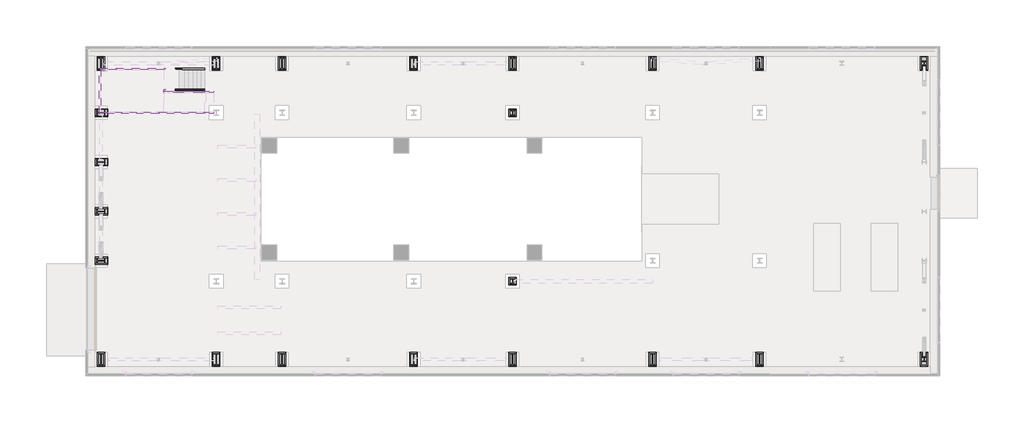
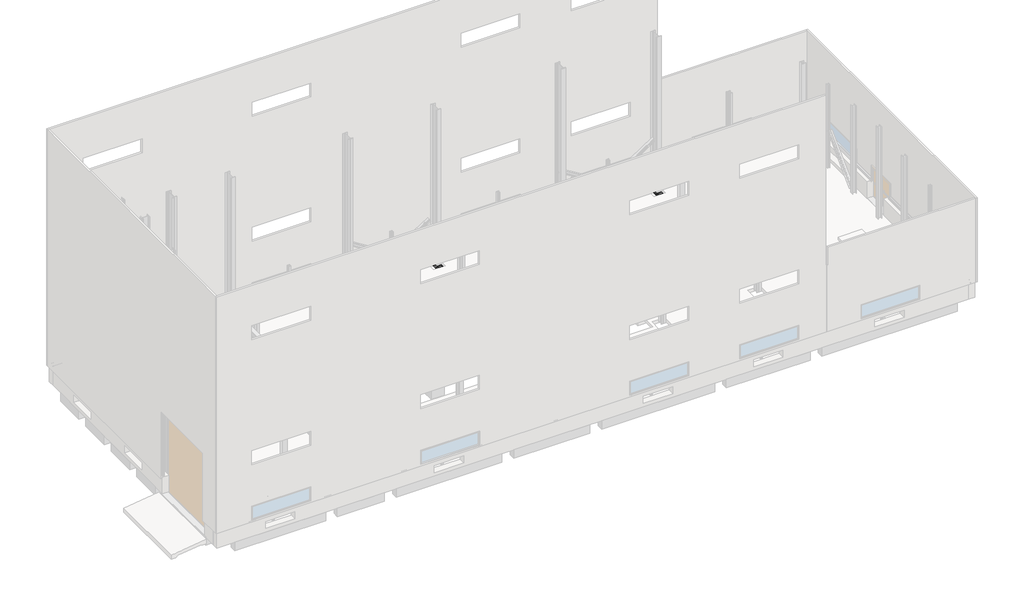
# One storey, part 4 of 4: 23 proxies, 10 members.
"""IFC4 building model written with IfcOpenShell, lengths in millimetres."""

import ifcopenshell
import ifcopenshell.guid

model = None  # the IFC model being written
_history = None  # IfcOwnerHistory: only IFC2X3 demands one
_inside = {}  # id of a spatial element -> (the spatial element, [elements in it])
_under = {}  # id of a project, library or spatial element -> (it, [spatial elements below it])
_declared = {}  # id of a project -> (the project, [libraries it declares])
_typed = {}  # id of a type object -> (the type object, [elements of that type])
_made_of = {}  # id of a material, layer set ... -> (it, [elements and type objects made of it])


def new_model(schema):
    """Start an empty IFC model of exactly this schema.

    Asked for "IFC4X3", IfcOpenShell would pick the latest addendum, in which some entities
    have other attributes; the version numbers below select the first issue.
    IFC2X3 requires an IfcOwnerHistory on every rooted entity: one is made here for all.
    """
    global model, _history
    if schema == "IFC4X3":
        model = ifcopenshell.file(schema_version=(4, 3, 0, 0))
    else:
        model = ifcopenshell.file(schema=schema)
    _inside.clear()
    _under.clear()
    _declared.clear()
    _typed.clear()
    _made_of.clear()
    _history = None
    if model.schema == "IFC2X3":
        org = make("IfcOrganization", Name="unknown")
        user = make(
            "IfcPersonAndOrganization",
            ThePerson=make("IfcPerson", FamilyName="unknown"),
            TheOrganization=org,
        )
        app = make(
            "IfcApplication",
            ApplicationDeveloper=org,
            Version="unknown",
            ApplicationFullName="unknown",
            ApplicationIdentifier="unknown",
        )
        _history = make(
            "IfcOwnerHistory",
            OwningUser=user,
            OwningApplication=app,
            ChangeAction="ADDED",
            CreationDate=0,
        )
    return model


def make(cls, **values):
    """One entity of the class cls with the attributes given. An attribute that is None is left unset."""
    return model.create_entity(
        cls, **{name: value for name, value in values.items() if value is not None}
    )


def rooted(cls, **values):
    """An entity with a GlobalId (a new one), such as an element, a storey or a relation."""
    return make(cls, GlobalId=ifcopenshell.guid.new(), OwnerHistory=_history, **values)


def si_unit(unit_type, name, prefix=None):
    """IfcSIUnit, for example si_unit("LENGTHUNIT", "METRE", prefix="MILLI")."""
    return make("IfcSIUnit", UnitType=unit_type, Prefix=prefix, Name=name)


def assignment(units):
    """IfcUnitAssignment: the units of a project."""
    return None if units is None else make("IfcUnitAssignment", Units=units)


def point(xyz):
    """IfcCartesianPoint."""
    return None if xyz is None else make("IfcCartesianPoint", Coordinates=xyz)


def direction(xyz):
    """IfcDirection."""
    return None if xyz is None else make("IfcDirection", DirectionRatios=xyz)


def frame(location, z_axis=None, x_axis=None):
    """IfcAxis2Placement3D, a coordinate frame: its origin and axes. An axis left out is left unset."""
    return make(
        "IfcAxis2Placement3D",
        Location=point(location),
        Axis=direction(z_axis),
        RefDirection=direction(x_axis),
    )


def frame_2d(location, x_axis=None):
    """IfcAxis2Placement2D, a coordinate frame in the plane: its origin and x axis."""
    return make(
        "IfcAxis2Placement2D", Location=point(location), RefDirection=direction(x_axis)
    )


def origin():
    """The frame at (0, 0, 0) with its axes left unset."""
    return frame((0.0, 0.0, 0.0))


def place(relative_to, where):
    """IfcLocalPlacement: puts the frame where relative to a parent placement (None: the world)."""
    return make(
        "IfcLocalPlacement", PlacementRelTo=relative_to, RelativePlacement=where
    )


def context(
    kind, dimensions, precision=None, world=None, true_north=None, identifier=None
):
    """IfcGeometricRepresentationContext, for example the 3D "Model" context."""
    return make(
        "IfcGeometricRepresentationContext",
        ContextIdentifier=identifier,
        ContextType=kind,
        CoordinateSpaceDimension=dimensions,
        Precision=precision,
        WorldCoordinateSystem=world,
        TrueNorth=true_north,
    )


def project(units=None, contexts=None):
    """IfcProject with its units and contexts."""
    return rooted(
        "IfcProject",
        Name="project",
        RepresentationContexts=contexts,
        UnitsInContext=assignment(units),
    )


def spatial(cls, under=None, at=None, **own):
    """A site, building, storey or space (cls), placed at a placement, below another one or the project."""
    s = rooted(cls, ObjectPlacement=at, **own)
    if under is not None:
        _under.setdefault(under.id(), (under, []))[1].append(s)
    return s


def polyline(points):
    """IfcPolyline through the points."""
    return make("IfcPolyline", Points=[point(p) for p in points])


def circle_curve(where, radius):
    """IfcCircle in the frame where."""
    return make("IfcCircle", Position=where, Radius=radius)


def ellipse_curve(where, semi_axis1, semi_axis2):
    """IfcEllipse in the frame where."""
    return make(
        "IfcEllipse", Position=where, SemiAxis1=semi_axis1, SemiAxis2=semi_axis2
    )


def trimmed(basis, trim1, trim2, sense, master):
    """IfcTrimmedCurve: the piece of a basis curve between two trims."""
    return make(
        "IfcTrimmedCurve",
        BasisCurve=basis,
        Trim1=trim1,
        Trim2=trim2,
        SenseAgreement=sense,
        MasterRepresentation=master,
    )


def segment(curve, same_sense, transition):
    """IfcCompositeCurveSegment."""
    return make(
        "IfcCompositeCurveSegment",
        Transition=transition,
        SameSense=same_sense,
        ParentCurve=curve,
    )


def composite_curve(segments, self_intersect=None):
    """IfcCompositeCurve: segments joined end to end."""
    return make("IfcCompositeCurve", Segments=segments, SelfIntersect=self_intersect)


def outline(outer, holes=None, kind="AREA"):
    """IfcArbitraryClosedProfileDef: a profile drawn as a closed curve; with holes, ...WithVoids."""
    if holes is None:
        return make("IfcArbitraryClosedProfileDef", ProfileType=kind, OuterCurve=outer)
    return make(
        "IfcArbitraryProfileDefWithVoids",
        ProfileType=kind,
        OuterCurve=outer,
        InnerCurves=holes,
    )


def extrude(swept, where, along, depth):
    """IfcExtrudedAreaSolid: the profile swept, set in the frame where, extruded along a direction by depth."""
    return make(
        "IfcExtrudedAreaSolid",
        SweptArea=swept,
        Position=where,
        ExtrudedDirection=direction(along),
        Depth=depth,
    )


def faces_of(points, faces, orient=None, outer=None):
    """IfcFace entities. A face is a list of loops; a loop is a list of indices into points, from 0.

    orient and outer hold one flag for each loop. By default every Orientation is true, the
    first loop of a face is its IfcFaceOuterBound and the others are IfcFaceBound.
    """
    made = []
    for i, loops in enumerate(faces):
        bounds = []
        for j, loop in enumerate(loops):
            is_outer = j == 0 if outer is None else outer[i][j]
            bounds.append(
                make(
                    "IfcFaceOuterBound" if is_outer else "IfcFaceBound",
                    Bound=make("IfcPolyLoop", Polygon=[points[k] for k in loop]),
                    Orientation=True if orient is None else orient[i][j],
                )
            )
        made.append(make("IfcFace", Bounds=bounds))
    return made


def faceted_brep(points, faces, orient=None, outer=None, voids=None):
    """IfcFacetedBrep: a solid bounded by flat faces; with voids (closed shells), ...WithVoids."""
    shared = [point(p) for p in points]
    hull = make("IfcClosedShell", CfsFaces=faces_of(shared, faces, orient, outer))
    if voids is None:
        return make("IfcFacetedBrep", Outer=hull)
    return make(
        "IfcFacetedBrepWithVoids",
        Outer=hull,
        Voids=[
            make(cls, CfsFaces=faces_of(shared, fs, o, b)) for cls, fs, o, b in voids
        ],
    )


def shape(context_of_items, identifier, shape_type, items):
    """IfcShapeRepresentation: the items that make up one representation, for example the "Body"."""
    return make(
        "IfcShapeRepresentation",
        ContextOfItems=context_of_items,
        RepresentationIdentifier=identifier,
        RepresentationType=shape_type,
        Items=items,
    )


def source(mapping_origin, context_of_items, identifier, shape_type, items):
    """IfcRepresentationMap: a shape defined once, which mapped items show again and again."""
    return make(
        "IfcRepresentationMap",
        MappingOrigin=mapping_origin,
        MappedRepresentation=shape(context_of_items, identifier, shape_type, items),
    )


def transform(
    local_origin,
    x_axis=None,
    y_axis=None,
    z_axis=None,
    scale=None,
    scale2=None,
    scale3=None,
    uniform=True,
):
    """IfcCartesianTransformationOperator3D, or its non-uniform kind. x_axis, y_axis, z_axis: its Axis1, 2, 3."""
    if uniform:
        return make(
            "IfcCartesianTransformationOperator3D",
            Axis1=direction(x_axis),
            Axis2=direction(y_axis),
            LocalOrigin=point(local_origin),
            Scale=scale,
            Axis3=direction(z_axis),
        )
    return make(
        "IfcCartesianTransformationOperator3DnonUniform",
        Axis1=direction(x_axis),
        Axis2=direction(y_axis),
        LocalOrigin=point(local_origin),
        Scale=scale,
        Axis3=direction(z_axis),
        Scale2=scale2,
        Scale3=scale3,
    )


def mapped(mapping_source, mapping_target):
    """IfcMappedItem: shows the shape of a source again, moved by a transform."""
    return make(
        "IfcMappedItem", MappingSource=mapping_source, MappingTarget=mapping_target
    )


def made_of(thing, what):
    """Note that an element or type object is made of a material, layer set ...; save() writes the relation."""
    if what is not None:
        _made_of.setdefault(what.id(), (what, []))[1].append(thing)
    return thing


def element(
    cls,
    number,
    at=None,
    inside=None,
    cuts=None,
    type_object=None,
    material=None,
    context=None,
    identifier="Body",
    shape_type=None,
    held_by="IfcProductDefinitionShape",
    body=None,
    shapes=None,
    **own,
):
    """One element of the class cls, such as IfcWall. Its Tag is "e" and its number.

    at: its placement. inside: the storey or other place that contains it. cuts: it is an
    opening in that element (IfcRelVoidsElement). A single representation is given by context,
    identifier, shape_type and body (its items); several are given by shapes. held_by: the class
    of the entity that holds the representations. save() writes the other relations.
    """
    e = rooted(cls, Tag="e%d" % number, ObjectPlacement=at, **own)
    if body is not None:
        shapes = [shape(context, identifier, shape_type, body)]
    if shapes is not None:
        e.Representation = make(held_by, Representations=shapes)
    if inside is not None:
        _inside.setdefault(inside.id(), (inside, []))[1].append(e)
    if cuts is not None:
        rooted(
            "IfcRelVoidsElement", RelatingBuildingElement=cuts, RelatedOpeningElement=e
        )
    if type_object is not None:
        _typed.setdefault(type_object.id(), (type_object, []))[1].append(e)
    return made_of(e, material)


def aggregate(whole, parts):
    """IfcRelAggregates: a whole, such as a stair, and the parts it consists of."""
    return rooted("IfcRelAggregates", RelatingObject=whole, RelatedObjects=parts)


def save(model, path):
    """Write the relations noted so far, then the file.

    IfcRelAggregates (storeys below a building ...), IfcRelContainedInSpatialStructure (elements
    in a storey), IfcRelDefinesByType, IfcRelAssociatesMaterial and IfcRelDeclares: one each for
    every whole, place, type object, material and project.
    """
    for whole, parts in _under.values():
        aggregate(whole, parts)
    for where, things in _inside.values():
        rooted(
            "IfcRelContainedInSpatialStructure",
            RelatedElements=things,
            RelatingStructure=where,
        )
    for kind, things in _typed.values():
        rooted("IfcRelDefinesByType", RelatedObjects=things, RelatingType=kind)
    for what, things in _made_of.values():
        rooted("IfcRelAssociatesMaterial", RelatedObjects=things, RelatingMaterial=what)
    for by, libraries in _declared.values():
        rooted("IfcRelDeclares", RelatingContext=by, RelatedDefinitions=libraries)
    model.write(path)


def plane_surface(at):
    """IfcPlane: the flat surface through the origin of the frame at, square to its z axis."""
    return make("IfcPlane", Position=at)


def cylinder_surface(at, radius):
    """IfcCylindricalSurface: all points at the distance radius from the z axis of the frame at."""
    return make("IfcCylindricalSurface", Position=at, Radius=radius)


def advanced_brep(points, edges, surfaces, faces):
    """IfcAdvancedBrep: a solid bounded by faces that lie on surfaces and meet in shared edges.

    An edge is (start, end): straight between two places in points (the first is 0);
    or (start, end, curve); or (start, end, curve, False) where it runs against its curve.
    A face is (place in surfaces, loops), or (place, loops, False) where it looks against
    its surface's normal. A loop lists edges by number (the first is 1), with a minus sign
    where the edge is run from its end to its start. The first loop is the outer one.
    """
    corners = [point(p) for p in points]
    vertices = [make("IfcVertexPoint", VertexGeometry=c) for c in corners]
    made = []
    for start, end, *more in edges:
        made.append(
            make(
                "IfcEdgeCurve",
                EdgeStart=vertices[start],
                EdgeEnd=vertices[end],
                EdgeGeometry=more[0] if more else make("IfcPolyline", Points=[corners[start], corners[end]]),
                SameSense=more[1] if len(more) > 1 else True,
            )
        )
    hull = []
    for where, loops, *sense in faces:
        bounds = []
        for j, loop in enumerate(loops):
            ring = [make("IfcOrientedEdge", EdgeElement=made[abs(k) - 1], Orientation=k > 0) for k in loop]
            bounds.append(
                make(
                    "IfcFaceOuterBound" if j == 0 else "IfcFaceBound",
                    Bound=make("IfcEdgeLoop", EdgeList=ring),
                    Orientation=True,
                )
            )
        hull.append(make("IfcAdvancedFace", Bounds=bounds, FaceSurface=surfaces[where], SameSense=sense[0] if sense else True))
    return make("IfcAdvancedBrep", Outer=make("IfcClosedShell", CfsFaces=hull))


def grout_43c68623(model_context):
    return source(origin(), model_context, "Body", "Brep", [
        faceted_brep([(175.0, 375.0, 863.9720055), (-175.0, 375.0, 863.9720055), (-175.0, -375.0, 863.9720055), (175.0, -375.0, 863.9720055), (225.0, 425.0, 813.9720055), (225.0, -425.0, 813.9720055), (-225.0, -425.0, 813.9720055), (-225.0, 425.0, 813.9720055)], [[[0, 1, 2, 3]], [[4, 5, 6, 7]], [[4, 7, 1, 0]], [[7, 6, 2, 1]], [[6, 5, 3, 2]], [[5, 4, 0, 3]]]),
    ])


def generic_models_49ee4eb4(model_context):
    return source(origin(), model_context, "Body", "Brep", [
        faceted_brep([(25169.0, 25924.5208589, 743.9720055), (24819.0, 25924.5208589, 743.9720055), (24819.0, 25574.5208589, 743.9720055), (25169.0, 25574.5208589, 743.9720055), (25219.0, 25974.5208589, 693.9720055), (25219.0, 25524.5208589, 693.9720055), (24769.0, 25524.5208589, 693.9720055), (24769.0, 25974.5208589, 693.9720055)], [[[0, 1, 2, 3]], [[4, 5, 6, 7]], [[4, 7, 1, 0]], [[7, 6, 2, 1]], [[6, 5, 3, 2]], [[5, 4, 0, 3]]]),
    ])


model = new_model("IFC4")

# Units and contexts
model_context = context("Model", 3, world=origin())
ifc_project = project(units=[si_unit("LENGTHUNIT", "METRE", prefix="MILLI")], contexts=[model_context])

# Site, building, storey
site = spatial("IfcSite", under=ifc_project)
building = spatial("IfcBuilding", under=site)
storey = spatial("IfcBuildingStorey", under=building, Name="1ST T.O.C", Elevation=599.9720055)

# Proxies
placement = place(None, origin())
grout_shape = grout_43c68623(model_context)
element("IfcBuildingElementProxy", 1, Name="그라우트 : 그라우트", ObjectType="그라우트 : 그라우트", at=placement, inside=storey, context=model_context, shape_type="MappedRepresentation", body=[
    mapped(grout_shape, transform((0.0, 20999.5208589, -214.0), x_axis=(1.0, 0.0, 0.0), y_axis=(0.0, 1.0, 0.0), z_axis=(0.0, 0.0, 1.0))),
])
element("IfcBuildingElementProxy", 2, Name="그라우트2 : 그라우트", ObjectType="그라우트2 : 그라우트", at=placement, inside=storey, context=model_context, shape_type="MappedRepresentation", body=[
    mapped(grout_shape, transform((6994.0, 20999.5208589, -214.0), x_axis=(1.0, 0.0, 0.0), y_axis=(0.0, 1.0, 0.0), z_axis=(0.0, 0.0, 1.0))),
])
element("IfcBuildingElementProxy", 3, Name="그라우트3 : 그라우트", ObjectType="그라우트3 : 그라우트", at=placement, inside=storey, context=model_context, shape_type="MappedRepresentation", body=[
    mapped(grout_shape, transform((10994.0, 20999.5208589, -214.0), x_axis=(1.0, 0.0, 0.0), y_axis=(0.0, 1.0, 0.0), z_axis=(0.0, 0.0, 1.0))),
])
element("IfcBuildingElementProxy", 4, Name="그라우트4 : 그라우트", ObjectType="그라우트4 : 그라우트", at=placement, inside=storey, context=model_context, shape_type="MappedRepresentation", body=[
    mapped(grout_shape, transform((18994.0, 20999.5208589, -214.0), x_axis=(1.0, 0.0, 0.0), y_axis=(0.0, 1.0, 0.0), z_axis=(0.0, 0.0, 1.0))),
])
element("IfcBuildingElementProxy", 5, Name="그라우트5 : 그라우트", ObjectType="그라우트5 : 그라우트", at=placement, inside=storey, context=model_context, shape_type="MappedRepresentation", body=[
    mapped(grout_shape, transform((24994.0, 20999.5208589, -214.0), x_axis=(1.0, 0.0, 0.0), y_axis=(0.0, 1.0, 0.0), z_axis=(0.0, 0.0, 1.0))),
])
element("IfcBuildingElementProxy", 6, Name="그라우트6 : 그라우트", ObjectType="그라우트6 : 그라우트", at=placement, inside=storey, context=model_context, shape_type="MappedRepresentation", body=[
    mapped(grout_shape, transform((33494.0, 20999.5208589, -214.0), x_axis=(1.0, 0.0, 0.0), y_axis=(0.0, 1.0, 0.0), z_axis=(0.0, 0.0, 1.0))),
])
element("IfcBuildingElementProxy", 7, Name="그라우트7 : 그라우트", ObjectType="그라우트7 : 그라우트", at=placement, inside=storey, context=model_context, shape_type="MappedRepresentation", body=[
    mapped(grout_shape, transform((39994.0, 20999.5208589, -214.0), x_axis=(1.0, 0.0, 0.0), y_axis=(0.0, 1.0, 0.0), z_axis=(0.0, 0.0, 1.0))),
])
element("IfcBuildingElementProxy", 8, Name="그라우트8 : 그라우트", ObjectType="그라우트8 : 그라우트", at=placement, inside=storey, context=model_context, shape_type="MappedRepresentation", body=[
    mapped(grout_shape, transform((39994.0, 38999.5208589, -214.0), x_axis=(1.0, 0.0, 0.0), y_axis=(0.0, 1.0, 0.0), z_axis=(0.0, 0.0, 1.0))),
])
element("IfcBuildingElementProxy", 9, Name="그라우트9 : 그라우트", ObjectType="그라우트9 : 그라우트", at=placement, inside=storey, context=model_context, shape_type="MappedRepresentation", body=[
    mapped(grout_shape, transform((33494.0, 38999.5208589, -214.0), x_axis=(1.0, 0.0, 0.0), y_axis=(0.0, 1.0, 0.0), z_axis=(0.0, 0.0, 1.0))),
])
element("IfcBuildingElementProxy", 10, Name="그라우트10 : 그라우트", ObjectType="그라우트10 : 그라우트", at=placement, inside=storey, context=model_context, shape_type="MappedRepresentation", body=[
    mapped(grout_shape, transform((24994.0, 38999.5208589, -214.0), x_axis=(1.0, 0.0, 0.0), y_axis=(0.0, 1.0, 0.0), z_axis=(0.0, 0.0, 1.0))),
])
element("IfcBuildingElementProxy", 11, Name="그라우트11 : 그라우트", ObjectType="그라우트11 : 그라우트", at=placement, inside=storey, context=model_context, shape_type="MappedRepresentation", body=[
    mapped(grout_shape, transform((18994.0, 38999.5208589, -214.0), x_axis=(1.0, 0.0, 0.0), y_axis=(0.0, 1.0, 0.0), z_axis=(0.0, 0.0, 1.0))),
])
element("IfcBuildingElementProxy", 12, Name="그라우트12 : 그라우트", ObjectType="그라우트12 : 그라우트", at=placement, inside=storey, context=model_context, shape_type="MappedRepresentation", body=[
    mapped(grout_shape, transform((10994.0, 38999.5208589, -214.0), x_axis=(1.0, 0.0, 0.0), y_axis=(0.0, 1.0, 0.0), z_axis=(0.0, 0.0, 1.0))),
])
element("IfcBuildingElementProxy", 13, Name="그라우트13 : 그라우트", ObjectType="그라우트13 : 그라우트", at=placement, inside=storey, context=model_context, shape_type="MappedRepresentation", body=[
    mapped(grout_shape, transform((6994.0, 38999.5208589, -214.0), x_axis=(1.0, 0.0, 0.0), y_axis=(0.0, 1.0, 0.0), z_axis=(0.0, 0.0, 1.0))),
])
element("IfcBuildingElementProxy", 14, Name="그라우트14 : 그라우트", ObjectType="그라우트14 : 그라우트", at=placement, inside=storey, context=model_context, shape_type="MappedRepresentation", body=[
    mapped(grout_shape, transform((-6.0, 38999.5208589, -214.0), x_axis=(1.0, 0.0, 0.0), y_axis=(0.0, 1.0, 0.0), z_axis=(0.0, 0.0, 1.0))),
])
element("IfcBuildingElementProxy", 15, Name="그라우트15 : 그라우트", ObjectType="그라우트15 : 그라우트", at=placement, inside=storey, context=model_context, shape_type="MappedRepresentation", body=[
    mapped(grout_shape, transform((-6.0, 35999.5208589, -214.0), x_axis=(0.0, -1.0, 0.0), y_axis=(1.0, 0.0, 0.0), z_axis=(0.0, 0.0, 1.0))),
])
element("IfcBuildingElementProxy", 16, Name="그라우트16 : 그라우트", ObjectType="그라우트16 : 그라우트", at=placement, inside=storey, context=model_context, shape_type="MappedRepresentation", body=[
    mapped(grout_shape, transform((-6.0, 32999.5208589, -214.0), x_axis=(0.0, -1.0, 0.0), y_axis=(1.0, 0.0, 0.0), z_axis=(0.0, 0.0, 1.0))),
])
element("IfcBuildingElementProxy", 17, Name="그라우트17 : 그라우트", ObjectType="그라우트17 : 그라우트", at=placement, inside=storey, context=model_context, shape_type="MappedRepresentation", body=[
    mapped(grout_shape, transform((-6.0, 29999.5208589, -214.0), x_axis=(0.0, -1.0, 0.0), y_axis=(1.0, 0.0, 0.0), z_axis=(0.0, 0.0, 1.0))),
])
element("IfcBuildingElementProxy", 18, Name="그라우트18 : 그라우트", ObjectType="그라우트18 : 그라우트", at=placement, inside=storey, context=model_context, shape_type="MappedRepresentation", body=[
    mapped(grout_shape, transform((-6.0, 26999.5208589, -214.0), x_axis=(0.0, -1.0, 0.0), y_axis=(1.0, 0.0, 0.0), z_axis=(0.0, 0.0, 1.0))),
])
element("IfcBuildingElementProxy", 19, Name="그라우트20 : 그라우트", ObjectType="그라우트20 : 그라우트", at=placement, inside=storey, context=model_context, shape_type="MappedRepresentation", body=[
    mapped(grout_shape, transform((49994.0, 38999.5208589, -214.0), x_axis=(1.0, 0.0, 0.0), y_axis=(0.0, 1.0, 0.0), z_axis=(0.0, 0.0, 1.0))),
])
element("IfcBuildingElementProxy", 20, Name="그라우트22 : 그라우트", ObjectType="그라우트22 : 그라우트", at=placement, inside=storey, context=model_context, shape_type="MappedRepresentation", body=[
    mapped(grout_shape, transform((49994.0, 20999.5208589, -214.0), x_axis=(1.0, 0.0, 0.0), y_axis=(0.0, 1.0, 0.0), z_axis=(0.0, 0.0, 1.0))),
])
generic_models_shape = generic_models_49ee4eb4(model_context)
element("IfcBuildingElementProxy", 21, Name="그라우트23 : 그라우트", ObjectType="그라우트23 : 그라우트", at=placement, inside=storey, context=model_context, shape_type="MappedRepresentation", body=[
    mapped(generic_models_shape, transform((0.0, 0.0, -94.0), x_axis=(1.0, 0.0, 0.0), y_axis=(0.0, 1.0, 0.0), z_axis=(0.0, 0.0, 1.0))),
])
element("IfcBuildingElementProxy", 22, Name="그라우트19 : 그라우트", ObjectType="그라우트19 : 그라우트", at=placement, inside=storey, context=model_context, shape_type="MappedRepresentation", body=[
    mapped(generic_models_shape, transform((0.0, 10250.0, -94.0), x_axis=(1.0, 0.0, 0.0), y_axis=(0.0, 1.0, 0.0), z_axis=(0.0, 0.0, 1.0))),
])
element("IfcBuildingElementProxy", 23, Name="Grout : H_GM_AMM_Grouting_T50", ObjectType="Grout : H_GM_AMM_Grouting_T50", at=placement, inside=storey, context=model_context, shape_type="MappedRepresentation", body=[
    mapped(grout_shape, transform((6994.0, 20999.5208589, -214.0), x_axis=(1.0, 0.0, 0.0), y_axis=(0.0, 1.0, 0.0), z_axis=(0.0, 0.0, 1.0))),
])

# Members
element("IfcMember", 24, ObjectType="C-250X90", at=placement, inside=storey, context=model_context, shape_type="AdvancedBrep", body=[
    advanced_brep(
    [(6309.5374538, 37424.5208589, 599.9720055), (6309.5374538, 37413.5208589, 599.9720055), (6192.9345962, 37413.5208589, 599.9720055), (6174.6503035, 37345.6208589, 599.9720055), (6155.7782632, 37334.5208589, 599.9720055), (6155.7782632, 37424.5208589, 599.9720055), (6309.5374538, 37424.5208589, 797.2714693), (6309.5374538, 37334.5208589, 797.2714693), (6309.5374538, 37345.6208589, 783.5463491), (6309.5374538, 37413.5208589, 770.2486816), (3899.5374538, 37424.5208589, 2240.8744123), (3899.5374538, 37424.5208589, 2549.998742), (3899.5374538, 37345.6208589, 2536.2736218), (3899.5374538, 37413.5208589, 2522.9759544), (3899.5374538, 37334.5208589, 2549.998742), (3899.5374538, 37334.5208589, 2240.8744123), (3899.5374538, 37345.6208589, 2254.5995325), (3899.5374538, 37413.5208589, 2267.8972)],
    [
        (0, 1),
        (1, 2),
        (2, 3),
        (3, 4, ellipse_curve(frame((6155.7782632, 37345.6208589, 599.9720055), z_axis=(0.0, 0.0, -1.0), x_axis=(1.0, 0.0, 0.0)), 18.8720403, 11.1)),
        (4, 5),
        (5, 0),
        (6, 7),
        (7, 8, ellipse_curve(frame((6309.5374538, 37345.6208589, 797.2714693), z_axis=(1.0, 0.0, 0.0), x_axis=(0.0, 0.0, -0.9999999999999999)), 13.7251202, 11.1)),
        (8, 9),
        (9, 1),
        (0, 6),
        (5, 10),
        (10, 11),
        (11, 6),
        (8, 12),
        (12, 13),
        (13, 9),
        (7, 14),
        (14, 12, ellipse_curve(frame((3899.5374538, 37345.6208589, 2549.998742), z_axis=(1.0, 0.0, 0.0), x_axis=(0.0, 0.0, -0.9999999999999999)), 13.7251202, 11.1)),
        (11, 14),
        (4, 15),
        (15, 10),
        (3, 16),
        (16, 15, ellipse_curve(frame((3899.5374538, 37345.6208589, 2240.8744123), z_axis=(1.0, 0.0, 0.0), x_axis=(0.0, 0.0, -0.9999999999999999)), 13.7251202, 11.1)),
        (2, 17),
        (17, 16),
        (13, 17),
    ],
    [
        plane_surface(frame((0.0, 0.0, 599.9720055), z_axis=(0.0, 0.0, -1.0), x_axis=(1.0, 0.0, 0.0))),
        plane_surface(frame((6309.5374538, 37424.5208589, 797.2714693), z_axis=(1.0, 0.0, 0.0), x_axis=(0.0, -1.0, 0.0))),
        plane_surface(frame((6309.5374538, 37424.5208589, 488.1471396), z_axis=(0.0, 1.0, 0.0), x_axis=(-0.8087360843031884, 0.0, 0.5881716976750463))),
        plane_surface(frame((6309.5374538, 37345.6208589, 783.5463491), z_axis=(-0.5809303280616924, -0.15643446504022573, -0.7987792010848263), x_axis=(-0.8087360843031886, 0.0, 0.5881716976750463))),
        cylinder_surface(frame((6309.5374538, 37345.6208589, 797.2714693), z_axis=(0.8087360843031884, 0.0, -0.5881716976750463), x_axis=(0.0, -1.0, 0.0)), 11.1),
        plane_surface(frame((6309.5374538, 37424.5208589, 797.2714693), z_axis=(0.5881716976750463, 0.0, 0.8087360843031886), x_axis=(-0.8087360843031886, 0.0, 0.5881716976750463))),
        plane_surface(frame((6309.5374538, 37334.5208589, 488.1471396), z_axis=(-0.5881716976750463, 0.0, -0.8087360843031884), x_axis=(-0.8087360843031884, 0.0, 0.5881716976750463))),
        cylinder_surface(frame((6162.4945294, 37345.6208589, 595.0874482), z_axis=(0.8087360843031884, 0.0, -0.5881716976750463), x_axis=(0.0, -1.0, 0.0)), 11.1),
        plane_surface(frame((6309.5374538, 37413.5208589, 515.1699273), z_axis=(0.5809303280616908, -0.15643446504023575, 0.7987792010848253), x_axis=(-0.8087360843031884, 0.0, 0.5881716976750463))),
        plane_surface(frame((6309.5374538, 37413.5208589, 770.2486816), z_axis=(0.0, -1.0, 0.0), x_axis=(-0.8087360843031884, 0.0, 0.5881716976750463))),
        plane_surface(frame((3899.5374538, 37328.5647627, 2426.9720055), z_axis=(-1.0, 0.0, 0.0), x_axis=(0.0, 1.0, 0.0))),
    ],
    [
        (0, [[1, 2, 3, 4, 5, 6]]),
        (1, [[7, 8, 9, 10, -1, 11]]),
        (2, [[-11, -6, 12, 13, 14]]),
        (3, [[-9, 15, 16, 17]]),
        (4, [[-8, 18, 19, -15]]),
        (5, [[-7, -14, 20, -18]]),
        (6, [[21, 22, -12, -5]]),
        (7, [[23, 24, -21, -4]]),
        (8, [[25, 26, -23, -3]]),
        (9, [[-10, -17, 27, -25, -2]]),
        (10, [[-13, -22, -24, -26, -27, -16, -19, -20]]),
    ],
),
])
element("IfcMember", 25, ObjectType="C-250X90", at=placement, inside=storey, context=model_context, shape_type="AdvancedBrep", body=[
    advanced_brep(
    [(6309.5374538, 38635.5208589, 599.9720055), (6309.5374538, 38624.5208589, 599.9720055), (6155.7782632, 38624.5208589, 599.9720055), (6155.7782632, 38714.5208589, 599.9720055), (6174.6503035, 38703.4208589, 599.9720055), (6192.9345962, 38635.5208589, 599.9720055), (6309.5374538, 38624.5208589, 797.2714693), (6309.5374538, 38635.5208589, 770.2486816), (6309.5374538, 38703.4208589, 783.5463491), (6309.5374538, 38714.5208589, 797.2714693), (3899.5742166, 38624.5208589, 2549.9720055), (3818.2782632, 38624.5208589, 2299.9720055), (3899.5742166, 38714.5208589, 2549.9720055), (3895.9646762, 38703.4208589, 2538.8720055), (3892.4675508, 38635.5208589, 2528.117702), (3818.2782632, 38714.5208589, 2299.9720055), (3821.8878035, 38703.4208589, 2311.0720055), (3825.3849289, 38635.5208589, 2321.826309)],
    [
        (0, 1),
        (1, 2),
        (2, 3),
        (3, 4, ellipse_curve(frame((6155.7782632, 38703.4208589, 599.9720055), z_axis=(0.0, 0.0, -1.0), x_axis=(1.0, 0.0, 0.0)), 18.8720403, 11.1)),
        (4, 5),
        (5, 0),
        (6, 1),
        (0, 7),
        (7, 8),
        (8, 9, ellipse_curve(frame((6309.5374538, 38703.4208589, 797.2714693), z_axis=(1.0, 0.0, 0.0), x_axis=(0.0, 0.0, -0.9999999999999999)), 13.7251202, 11.1)),
        (9, 6),
        (6, 10),
        (10, 11),
        (11, 2),
        (9, 12),
        (12, 10),
        (8, 13),
        (13, 12, ellipse_curve(frame((3899.5742166, 38703.4208589, 2549.9720055), z_axis=(0.9509826718461247, 0.0, -0.30924417189076664), x_axis=(-0.30924417189076714, 0.0, -0.9509826718461244)), 11.672137, 11.1)),
        (7, 14),
        (14, 13),
        (11, 15),
        (15, 3),
        (4, 16),
        (16, 17),
        (17, 5),
        (15, 16, ellipse_curve(frame((3818.2782632, 38703.4208589, 2299.9720055), z_axis=(0.9509826718461247, 0.0, -0.30924417189076664), x_axis=(-0.30924417189076714, 0.0, -0.9509826718461244)), 11.672137, 11.1)),
        (17, 14),
    ],
    [
        plane_surface(frame((0.0, 0.0, 599.9720055), z_axis=(0.0, 0.0, -1.0), x_axis=(1.0, 0.0, 0.0))),
        plane_surface(frame((6309.5374538, 38624.5208589, 797.2714693), z_axis=(1.0, 0.0, 0.0), x_axis=(0.0, -1.0, 0.0))),
        plane_surface(frame((6309.5374538, 38624.5208589, 797.2714693), z_axis=(0.0, -1.0000000000000002, 0.0), x_axis=(-0.8087360843031886, 0.0, 0.5881716976750463))),
        plane_surface(frame((6309.5374538, 38714.5208589, 797.2714693), z_axis=(0.5881716976750463, 0.0, 0.8087360843031886), x_axis=(-0.8087360843031886, 0.0, 0.5881716976750463))),
        cylinder_surface(frame((6309.5374538, 38703.4208589, 797.2714693), z_axis=(0.8087360843031884, 0.0, -0.5881716976750463), x_axis=(0.0, 1.0, 0.0)), 11.1),
        plane_surface(frame((6309.5374538, 38635.5208589, 770.2486816), z_axis=(-0.5809303280616913, 0.15643446504022976, -0.798779201084826), x_axis=(-0.8087360843031884, 0.0, 0.5881716976750463))),
        plane_surface(frame((6309.5374538, 38624.5208589, 488.1471396), z_axis=(-0.5881716976750463, 0.0, -0.8087360843031884), x_axis=(-0.8087360843031884, 0.0, 0.5881716976750463))),
        plane_surface(frame((6309.5374538, 38703.4208589, 501.8722598), z_axis=(0.5809303280616918, 0.1564344650402317, 0.7987792010848254), x_axis=(-0.8087360843031884, 0.0, 0.5881716976750463))),
        cylinder_surface(frame((6162.4945294, 38703.4208589, 595.0874482), z_axis=(0.8087360843031884, 0.0, -0.5881716976750463), x_axis=(0.0, 1.0, 0.0)), 11.1),
        plane_surface(frame((6309.5374538, 38635.5208589, 515.1699273), z_axis=(0.0, 1.0000000000000002, 0.0), x_axis=(-0.8087360843031886, 0.0, 0.5881716976750463))),
        plane_surface(frame((3899.5742166, 38624.5208589, 2549.9720055), z_axis=(-0.9509826718461247, 0.0, 0.30924417189076664), x_axis=(0.0, 1.0, 0.0))),
    ],
    [
        (0, [[1, 2, 3, 4, 5, 6]]),
        (1, [[7, -1, 8, 9, 10, 11]]),
        (2, [[-7, 12, 13, 14, -2]]),
        (3, [[-11, 15, 16, -12]]),
        (4, [[-10, 17, 18, -15]]),
        (5, [[-9, 19, 20, -17]]),
        (6, [[-14, 21, 22, -3]]),
        (7, [[23, 24, 25, -5]]),
        (8, [[-22, 26, -23, -4]]),
        (9, [[-8, -6, -25, 27, -19]]),
        (10, [[-16, -18, -20, -27, -24, -26, -21, -13]]),
    ],
),
])
element("IfcMember", 26, ObjectType="C-250X90", at=placement, inside=storey, context=model_context, shape_type="AdvancedBrep", body=[
    advanced_brep(
    [(3809.5374538, 37232.6086665, 2797.2714693), (3809.5374538, 37232.6086665, 2488.1471396), (6300.7966445, 37232.6086665, 4299.9720055), (6219.5006911, 37232.6086665, 4549.9720055), (3809.5374538, 37322.6086665, 2488.1471396), (6300.7966445, 37322.6086665, 4299.9720055), (3809.5374538, 37311.5086665, 2501.8722598), (6297.1871042, 37311.5086665, 4311.0720055), (3809.5374538, 37243.6086665, 2515.1699273), (6293.6899788, 37243.6086665, 4321.826309), (3809.5374538, 37243.6086665, 2770.2486816), (3809.5374538, 37311.5086665, 2783.5463491), (6223.1102315, 37311.5086665, 4538.8720055), (6226.6073569, 37243.6086665, 4528.117702), (3809.5374538, 37322.6086665, 2797.2714693), (6219.5006911, 37322.6086665, 4549.9720055)],
    [
        (0, 1),
        (1, 2),
        (2, 3),
        (3, 0),
        (1, 4),
        (4, 5),
        (5, 2),
        (4, 6, ellipse_curve(frame((3809.5374538, 37311.5086665, 2488.1471396), z_axis=(1.0, 0.0, 0.0), x_axis=(0.0, 0.0, -1.0)), 13.7251202, 11.1)),
        (6, 7),
        (7, 5, ellipse_curve(frame((6300.7966445, 37311.5086665, 4299.9720055), z_axis=(-0.9509826718461247, 0.0, -0.30924417189076625), x_axis=(0.3092441718907662, 0.0, -0.9509826718461247)), 11.672137, 11.1)),
        (6, 8),
        (8, 9),
        (9, 7),
        (10, 11),
        (11, 12),
        (12, 13),
        (13, 10),
        (11, 14, ellipse_curve(frame((3809.5374538, 37311.5086665, 2797.2714693), z_axis=(1.0, 0.0, 0.0), x_axis=(0.0, 0.0, -1.0)), 13.7251202, 11.1)),
        (14, 15),
        (15, 12, ellipse_curve(frame((6219.5006911, 37311.5086665, 4549.9720055), z_axis=(-0.9509826718461247, 0.0, -0.30924417189076625), x_axis=(0.3092441718907662, 0.0, -0.9509826718461247)), 11.672137, 11.1)),
        (14, 0),
        (3, 15),
        (8, 10),
        (13, 9),
    ],
    [
        plane_surface(frame((3809.5374538, 37232.6086665, 2488.1471396), z_axis=(0.0, -1.0, 0.0), x_axis=(0.8087360843031883, 0.0, 0.5881716976750465))),
        plane_surface(frame((3809.5374538, 37322.6086665, 2488.1471396), z_axis=(0.5881716976750465, 0.0, -0.8087360843031883), x_axis=(0.8087360843031883, 0.0, 0.5881716976750465))),
        cylinder_surface(frame((3956.5803783, 37311.5086665, 2595.0874482), z_axis=(-0.8087360843031883, 0.0, -0.5881716976750465), x_axis=(0.0, 1.0, 0.0)), 11.1),
        plane_surface(frame((3809.5374538, 37243.6086665, 2515.1699273), z_axis=(-0.5809303280616911, 0.15643446504023578, 0.798779201084825), x_axis=(0.8087360843031882, 0.0, 0.5881716976750466))),
        plane_surface(frame((3809.5374538, 37311.5086665, 2783.5463491), z_axis=(0.5809303280616926, 0.15643446504022573, -0.798779201084826), x_axis=(0.8087360843031883, 0.0, 0.5881716976750465))),
        cylinder_surface(frame((3809.5374538, 37311.5086665, 2797.2714693), z_axis=(-0.8087360843031883, 0.0, -0.5881716976750465), x_axis=(0.0, 1.0, 0.0)), 11.1),
        plane_surface(frame((3809.5374538, 37232.6086665, 2797.2714693), z_axis=(-0.5881716976750465, 0.0, 0.8087360843031883), x_axis=(0.8087360843031883, 0.0, 0.5881716976750465))),
        plane_surface(frame((3809.5374538, 37243.6086665, 2770.2486816), z_axis=(0.0, 1.0, 0.0), x_axis=(0.8087360843031883, 0.0, 0.5881716976750465))),
        plane_surface(frame((3809.5374538, 37328.5647627, 2426.9720055), z_axis=(-1.0, 0.0, 0.0), x_axis=(0.0, 1.0, 0.0))),
        plane_surface(frame((6219.5006911, 37282.6086665, 4549.9720055), z_axis=(0.9509826718461247, 0.0, 0.30924417189076625), x_axis=(0.0, -1.0, 0.0))),
    ],
    [
        (0, [[1, 2, 3, 4]]),
        (1, [[5, 6, 7, -2]]),
        (2, [[8, 9, 10, -6]]),
        (3, [[11, 12, 13, -9]]),
        (4, [[14, 15, 16, 17]]),
        (5, [[18, 19, 20, -15]]),
        (6, [[21, -4, 22, -19]]),
        (7, [[23, -17, 24, -12]]),
        (8, [[-21, -18, -14, -23, -11, -8, -5, -1]]),
        (9, [[-3, -7, -10, -13, -24, -16, -20, -22]]),
    ],
),
])
element("IfcMember", 27, ObjectType="C-250X90", at=placement, inside=storey, context=model_context, shape_type="AdvancedBrep", body=[
    advanced_brep(
    [(3550.7966445, 36032.6086665, 2299.9720055), (3469.5006911, 36032.6086665, 2549.9720055), (6219.5006911, 36032.6086665, 4549.9720055), (6300.7966445, 36032.6086665, 4299.9720055), (3469.5006911, 35942.6086665, 2549.9720055), (6219.5006911, 35942.6086665, 4549.9720055), (3473.1102315, 35953.7086665, 2538.8720055), (6223.1102315, 35953.7086665, 4538.8720055), (3476.6073569, 36021.6086665, 2528.117702), (6226.6073569, 36021.6086665, 4528.117702), (3543.6899788, 36021.6086665, 2321.826309), (3547.1871042, 35953.7086665, 2311.0720055), (6297.1871042, 35953.7086665, 4311.0720055), (6293.6899788, 36021.6086665, 4321.826309), (3550.7966445, 35942.6086665, 2299.9720055), (6300.7966445, 35942.6086665, 4299.9720055)],
    [
        (0, 1),
        (1, 2),
        (2, 3),
        (3, 0),
        (1, 4),
        (4, 5),
        (5, 2),
        (4, 6, ellipse_curve(frame((3469.5006911, 35953.7086665, 2549.9720055), z_axis=(0.9509826718461252, 0.0, 0.30924417189076514), x_axis=(0.3092441718907655, 0.0, -0.9509826718461252)), 11.672137, 11.1)),
        (6, 7),
        (7, 5, ellipse_curve(frame((6219.5006911, 35953.7086665, 4549.9720055), z_axis=(-0.9509826718461247, 0.0, -0.30924417189076625), x_axis=(0.3092441718907662, 0.0, -0.9509826718461247)), 11.672137, 11.1)),
        (6, 8),
        (8, 9),
        (9, 7),
        (10, 11),
        (11, 12),
        (12, 13),
        (13, 10),
        (11, 14, ellipse_curve(frame((3550.7966445, 35953.7086665, 2299.9720055), z_axis=(0.9509826718461252, 0.0, 0.30924417189076514), x_axis=(0.3092441718907655, 0.0, -0.9509826718461252)), 11.672137, 11.1)),
        (14, 15),
        (15, 12, ellipse_curve(frame((6300.7966445, 35953.7086665, 4299.9720055), z_axis=(-0.9509826718461247, 0.0, -0.30924417189076625), x_axis=(0.3092441718907662, 0.0, -0.9509826718461247)), 11.672137, 11.1)),
        (14, 0),
        (3, 15),
        (8, 10),
        (13, 9),
    ],
    [
        plane_surface(frame((3809.5374538, 36032.6086665, 2797.2714693), z_axis=(0.0, 1.0, 0.0), x_axis=(0.8087360843031883, 0.0, 0.5881716976750465))),
        plane_surface(frame((3809.5374538, 35942.6086665, 2797.2714693), z_axis=(-0.5881716976750465, 0.0, 0.8087360843031883), x_axis=(0.8087360843031883, 0.0, 0.5881716976750465))),
        cylinder_surface(frame((3809.5374538, 35953.7086665, 2797.2714693), z_axis=(-0.8087360843031883, 0.0, -0.5881716976750465), x_axis=(0.0, -1.0, 0.0)), 11.1),
        plane_surface(frame((3809.5374538, 36021.6086665, 2770.2486816), z_axis=(0.5809303280616915, -0.1564344650402298, -0.7987792010848259), x_axis=(0.8087360843031883, 0.0, 0.5881716976750465))),
        plane_surface(frame((3809.5374538, 35953.7086665, 2501.8722598), z_axis=(-0.5809303280616922, -0.15643446504023178, 0.7987792010848251), x_axis=(0.8087360843031882, 0.0, 0.5881716976750466))),
        cylinder_surface(frame((3956.5803783, 35953.7086665, 2595.0874482), z_axis=(-0.8087360843031883, 0.0, -0.5881716976750465), x_axis=(0.0, -1.0, 0.0)), 11.1),
        plane_surface(frame((3809.5374538, 36032.6086665, 2488.1471396), z_axis=(0.5881716976750465, 0.0, -0.8087360843031883), x_axis=(0.8087360843031883, 0.0, 0.5881716976750465))),
        plane_surface(frame((3809.5374538, 36021.6086665, 2515.1699273), z_axis=(0.0, -1.0, 0.0), x_axis=(0.8087360843031882, 0.0, 0.5881716976750466))),
        plane_surface(frame((3469.5006911, 36032.6086665, 2549.9720055), z_axis=(-0.9509826718461252, 0.0, -0.30924417189076514), x_axis=(0.0, -1.0, 0.0))),
        plane_surface(frame((6219.5006911, 36032.6086665, 4549.9720055), z_axis=(0.9509826718461247, 0.0, 0.30924417189076625), x_axis=(0.0, -1.0, 0.0))),
    ],
    [
        (0, [[1, 2, 3, 4]]),
        (1, [[5, 6, 7, -2]]),
        (2, [[8, 9, 10, -6]]),
        (3, [[11, 12, 13, -9]]),
        (4, [[14, 15, 16, 17]]),
        (5, [[18, 19, 20, -15]]),
        (6, [[21, -4, 22, -19]]),
        (7, [[23, -17, 24, -12]]),
        (8, [[-1, -21, -18, -14, -23, -11, -8, -5]]),
        (9, [[-7, -10, -13, -24, -16, -20, -22, -3]]),
    ],
),
])
element("IfcMember", 28, ObjectType="C-250X90", at=placement, inside=storey, context=model_context, shape_type="SweptSolid", body=[
    extrude(outline(composite_curve([segment(polyline([(2549.9720055, 3809.5374538), (2299.9720055, 3809.5374538), (2299.9720055, 3899.5374538)]), True, "CONTINUOUS"), segment(trimmed(circle_curve(frame_2d((2299.9720055, 3888.4374538)), 11.1), [point((2299.9720055, 3899.5374538))], [point((2311.0720055, 3888.4374538))], False, "CARTESIAN"), True, "CONTINUOUS"), segment(polyline([(2311.0720055, 3888.4374538), (2321.826309, 3820.5374538), (2528.117702, 3820.5374538), (2538.8720055, 3888.4374538)]), True, "CONTINUOUS"), segment(trimmed(circle_curve(frame_2d((2549.9720055, 3888.4374538)), 11.1), [point((2538.8720055, 3888.4374538))], [point((2549.9720055, 3899.5374538))], False, "CARTESIAN"), True, "CONTINUOUS"), segment(polyline([(2549.9720055, 3899.5374538), (2549.9720055, 3809.5374538)]), True, "CONTINUOUS")], self_intersect=False)), frame((0.0, 37322.6086665, 0.0), z_axis=(0.0, 1.0, 0.0), x_axis=(0.0, 0.0, 1.0)), (0.0, 0.0, 1.0), 101.9121924),
])
element("IfcMember", 29, ObjectType="C-250X90", at=placement, inside=storey, context=model_context, shape_type="AdvancedBrep", body=[
    advanced_brep(
    [(3818.2782632, 38624.5208589, 2299.9720055), (3899.5742166, 38624.5208589, 2549.9720055), (0.0, 38624.5208589, 2549.9720055), (0.0, 38624.5208589, 2299.9720055), (3899.5742166, 38714.5208589, 2549.9720055), (-90.0, 38714.5208589, 2549.9720055), (3895.9646762, 38703.4208589, 2538.8720055), (-78.9, 38703.4208589, 2538.8720055), (3892.4675508, 38635.5208589, 2528.117702), (-11.0, 38635.5208589, 2528.117702), (3825.3849289, 38635.5208589, 2321.826309), (3821.8878035, 38703.4208589, 2311.0720055), (-78.9, 38703.4208589, 2311.0720055), (-11.0, 38635.5208589, 2321.826309), (3818.2782632, 38714.5208589, 2299.9720055), (-90.0, 38714.5208589, 2299.9720055)],
    [
        (0, 1),
        (1, 2),
        (2, 3),
        (3, 0),
        (1, 4),
        (4, 5),
        (5, 2),
        (4, 6, ellipse_curve(frame((3899.5742166, 38703.4208589, 2549.9720055), z_axis=(-0.9509826718461252, 0.0, 0.30924417189076514), x_axis=(0.30924417189076503, 0.0, 0.9509826718461252)), 11.672137, 11.1)),
        (6, 7),
        (7, 5, ellipse_curve(frame((-78.9, 38703.4208589, 2549.9720055), z_axis=(0.7071067811865591, 0.707106781186536, 0.0), x_axis=(0.7071067811865358, -0.7071067811865591, 0.0)), 15.6977705, 11.1)),
        (6, 8),
        (8, 9),
        (9, 7),
        (10, 11),
        (11, 12),
        (12, 13),
        (13, 10),
        (11, 14, ellipse_curve(frame((3818.2782632, 38703.4208589, 2299.9720055), z_axis=(-0.9509826718461252, 0.0, 0.30924417189076514), x_axis=(0.30924417189076503, 0.0, 0.9509826718461252)), 11.672137, 11.1)),
        (14, 15),
        (15, 12, ellipse_curve(frame((-78.9, 38703.4208589, 2299.9720055), z_axis=(0.7071067811865591, 0.707106781186536, 0.0), x_axis=(0.7071067811865358, -0.7071067811865591, 0.0)), 15.6977705, 11.1)),
        (14, 0),
        (3, 15),
        (8, 10),
        (13, 9),
    ],
    [
        plane_surface(frame((3809.5374538, 38624.5208589, 2549.9720055), z_axis=(0.0, -1.0, 0.0), x_axis=(-1.0, 0.0, 0.0))),
        plane_surface(frame((3809.5374538, 38714.5208589, 2549.9720055), z_axis=(0.0, 0.0, 1.0), x_axis=(-1.0, 0.0, 0.0))),
        cylinder_surface(frame((3809.5374538, 38703.4208589, 2549.9720055), z_axis=(1.0, 0.0, 0.0), x_axis=(0.0, 1.0, 0.0)), 11.1),
        plane_surface(frame((3809.5374538, 38635.5208589, 2528.117702), z_axis=(0.0, 0.15643446504022773, -0.9876883405951383), x_axis=(-1.0, 0.0, 0.0))),
        plane_surface(frame((3809.5374538, 38703.4208589, 2311.0720055), z_axis=(0.0, 0.15643446504023373, 0.9876883405951373), x_axis=(-1.0, 0.0, 0.0))),
        cylinder_surface(frame((3809.5374538, 38703.4208589, 2299.9720055), z_axis=(1.0, 0.0, 0.0), x_axis=(0.0, 1.0, 0.0)), 11.1),
        plane_surface(frame((3809.5374538, 38624.5208589, 2299.9720055), z_axis=(0.0, 0.0, -1.0), x_axis=(-1.0, 0.0, 0.0))),
        plane_surface(frame((3809.5374538, 38635.5208589, 2321.826309), z_axis=(0.0, 1.0, 0.0), x_axis=(-1.0, 0.0, 0.0))),
        plane_surface(frame((3899.5742166, 38624.5208589, 2549.9720055), z_axis=(0.9509826718461252, 0.0, -0.30924417189076514), x_axis=(0.0, 1.0, 0.0))),
        plane_surface(frame((0.0, 38624.5208589, 2549.9720055), z_axis=(-0.7071067811865591, -0.707106781186536, 0.0), x_axis=(-0.707106781186536, 0.7071067811865591, 0.0))),
    ],
    [
        (0, [[1, 2, 3, 4]]),
        (1, [[5, 6, 7, -2]]),
        (2, [[8, 9, 10, -6]]),
        (3, [[11, 12, 13, -9]]),
        (4, [[14, 15, 16, 17]]),
        (5, [[18, 19, 20, -15]]),
        (6, [[21, -4, 22, -19]]),
        (7, [[23, -17, 24, -12]]),
        (8, [[-1, -21, -18, -14, -23, -11, -8, -5]]),
        (9, [[-7, -10, -13, -24, -16, -20, -22, -3]]),
    ],
),
])
element("IfcMember", 30, ObjectType="C-250X90", at=placement, inside=storey, context=model_context, shape_type="AdvancedBrep", body=[
    advanced_brep(
    [(0.0, 38624.5208589, 2299.9720055), (0.0, 38624.5208589, 2549.9720055), (0.0, 36032.6086665, 2549.9720055), (0.0, 36032.6086665, 2299.9720055), (-90.0, 38714.5208589, 2549.9720055), (-90.0, 35942.6086665, 2549.9720055), (-78.9, 38703.4208589, 2538.8720055), (-78.9, 35953.7086665, 2538.8720055), (-11.0, 38635.5208589, 2528.117702), (-11.0, 36021.6086665, 2528.117702), (-11.0, 38635.5208589, 2321.826309), (-78.9, 38703.4208589, 2311.0720055), (-78.9, 35953.7086665, 2311.0720055), (-11.0, 36021.6086665, 2321.826309), (-90.0, 38714.5208589, 2299.9720055), (-90.0, 35942.6086665, 2299.9720055)],
    [
        (0, 1),
        (1, 2),
        (2, 3),
        (3, 0),
        (1, 4),
        (4, 5),
        (5, 2),
        (4, 6, ellipse_curve(frame((-78.9, 38703.4208589, 2549.9720055), z_axis=(-0.7071067811865591, -0.707106781186536, 0.0), x_axis=(-0.707106781186536, 0.7071067811865588, 0.0)), 15.6977705, 11.1)),
        (6, 7),
        (7, 5, ellipse_curve(frame((-78.9, 35953.7086665, 2549.9720055), z_axis=(-0.7071067811865591, 0.707106781186536, 0.0), x_axis=(0.707106781186536, 0.7071067811865588, 0.0)), 15.6977705, 11.1)),
        (6, 8),
        (8, 9),
        (9, 7),
        (10, 11),
        (11, 12),
        (12, 13),
        (13, 10),
        (11, 14, ellipse_curve(frame((-78.9, 38703.4208589, 2299.9720055), z_axis=(-0.7071067811865591, -0.707106781186536, 0.0), x_axis=(-0.707106781186536, 0.7071067811865588, 0.0)), 15.6977705, 11.1)),
        (14, 15),
        (15, 12, ellipse_curve(frame((-78.9, 35953.7086665, 2299.9720055), z_axis=(-0.7071067811865591, 0.707106781186536, 0.0), x_axis=(0.707106781186536, 0.7071067811865588, 0.0)), 15.6977705, 11.1)),
        (14, 0),
        (3, 15),
        (8, 10),
        (13, 9),
    ],
    [
        plane_surface(frame((0.0, 38624.5208589, 2549.9720055), z_axis=(1.0, 0.0, 0.0), x_axis=(0.0, -1.0, 0.0))),
        plane_surface(frame((-90.0, 38624.5208589, 2549.9720055), z_axis=(0.0, 0.0, 1.0), x_axis=(0.0, -1.0, 0.0))),
        cylinder_surface(frame((-78.9, 38624.5208589, 2549.9720055), z_axis=(0.0, 1.0, 0.0), x_axis=(-1.0, 0.0, 0.0)), 11.1),
        plane_surface(frame((-11.0, 38624.5208589, 2528.117702), z_axis=(-0.15643446504022773, 0.0, -0.9876883405951383), x_axis=(0.0, -1.0, 0.0))),
        plane_surface(frame((-78.9, 38624.5208589, 2311.0720055), z_axis=(-0.15643446504023373, 0.0, 0.9876883405951373), x_axis=(0.0, -1.0, 0.0))),
        cylinder_surface(frame((-78.9, 38624.5208589, 2299.9720055), z_axis=(0.0, 1.0, 0.0), x_axis=(-1.0, 0.0, 0.0)), 11.1),
        plane_surface(frame((0.0, 38624.5208589, 2299.9720055), z_axis=(0.0, 0.0, -1.0), x_axis=(0.0, -1.0, 0.0))),
        plane_surface(frame((-11.0, 38624.5208589, 2321.826309), z_axis=(-1.0, 0.0, 0.0), x_axis=(0.0, -1.0, 0.0))),
        plane_surface(frame((0.0, 38624.5208589, 2549.9720055), z_axis=(0.7071067811865591, 0.707106781186536, 0.0), x_axis=(-0.707106781186536, 0.7071067811865591, 0.0))),
        plane_surface(frame((0.0, 36032.6086665, 2549.9720055), z_axis=(0.7071067811865591, -0.707106781186536, 0.0), x_axis=(-0.707106781186536, -0.7071067811865591, 0.0))),
    ],
    [
        (0, [[1, 2, 3, 4]]),
        (1, [[5, 6, 7, -2]]),
        (2, [[8, 9, 10, -6]]),
        (3, [[11, 12, 13, -9]]),
        (4, [[14, 15, 16, 17]]),
        (5, [[18, 19, 20, -15]]),
        (6, [[21, -4, 22, -19]]),
        (7, [[23, -17, 24, -12]]),
        (8, [[-1, -21, -18, -14, -23, -11, -8, -5]]),
        (9, [[-7, -10, -13, -24, -16, -20, -22, -3]]),
    ],
),
])
element("IfcMember", 31, ObjectType="C-250X90", at=placement, inside=storey, context=model_context, shape_type="AdvancedBrep", body=[
    advanced_brep(
    [(0.0, 36032.6086665, 2299.9720055), (0.0, 36032.6086665, 2549.9720055), (3469.5006911, 36032.6086665, 2549.9720055), (3550.7966445, 36032.6086665, 2299.9720055), (-90.0, 35942.6086665, 2549.9720055), (3469.5006911, 35942.6086665, 2549.9720055), (-78.9, 35953.7086665, 2538.8720055), (3473.1102315, 35953.7086665, 2538.8720055), (-11.0, 36021.6086665, 2528.117702), (3476.6073569, 36021.6086665, 2528.117702), (-11.0, 36021.6086665, 2321.826309), (-78.9, 35953.7086665, 2311.0720055), (3547.1871042, 35953.7086665, 2311.0720055), (3543.6899788, 36021.6086665, 2321.826309), (-90.0, 35942.6086665, 2299.9720055), (3550.7966445, 35942.6086665, 2299.9720055)],
    [
        (0, 1),
        (1, 2),
        (2, 3),
        (3, 0),
        (1, 4),
        (4, 5),
        (5, 2),
        (4, 6, ellipse_curve(frame((-78.9, 35953.7086665, 2549.9720055), z_axis=(0.7071067811865591, -0.707106781186536, 0.0), x_axis=(-0.7071067811865358, -0.7071067811865591, 0.0)), 15.6977705, 11.1)),
        (6, 7),
        (7, 5, ellipse_curve(frame((3469.5006911, 35953.7086665, 2549.9720055), z_axis=(-0.9509826718461255, 0.0, -0.3092441718907639), x_axis=(-0.3092441718907641, 0.0, 0.9509826718461254)), 11.672137, 11.1)),
        (6, 8),
        (8, 9),
        (9, 7),
        (10, 11),
        (11, 12),
        (12, 13),
        (13, 10),
        (11, 14, ellipse_curve(frame((-78.9, 35953.7086665, 2299.9720055), z_axis=(0.7071067811865591, -0.707106781186536, 0.0), x_axis=(-0.7071067811865358, -0.7071067811865591, 0.0)), 15.6977705, 11.1)),
        (14, 15),
        (15, 12, ellipse_curve(frame((3550.7966445, 35953.7086665, 2299.9720055), z_axis=(-0.9509826718461255, 0.0, -0.3092441718907639), x_axis=(-0.3092441718907641, 0.0, 0.9509826718461254)), 11.672137, 11.1)),
        (14, 0),
        (3, 15),
        (8, 10),
        (13, 9),
    ],
    [
        plane_surface(frame((0.0, 36032.6086665, 2549.9720055), z_axis=(0.0, 1.0, 0.0), x_axis=(1.0, 0.0, 0.0))),
        plane_surface(frame((0.0, 35942.6086665, 2549.9720055), z_axis=(0.0, 0.0, 1.0), x_axis=(1.0, 0.0, 0.0))),
        cylinder_surface(frame((0.0, 35953.7086665, 2549.9720055), z_axis=(-1.0, 0.0, 0.0), x_axis=(0.0, -1.0, 0.0)), 11.1),
        plane_surface(frame((0.0, 36021.6086665, 2528.117702), z_axis=(0.0, -0.15643446504022773, -0.9876883405951383), x_axis=(1.0, 0.0, 0.0))),
        plane_surface(frame((0.0, 35953.7086665, 2311.0720055), z_axis=(0.0, -0.15643446504023373, 0.9876883405951373), x_axis=(1.0, 0.0, 0.0))),
        cylinder_surface(frame((0.0, 35953.7086665, 2299.9720055), z_axis=(-1.0, 0.0, 0.0), x_axis=(0.0, -1.0, 0.0)), 11.1),
        plane_surface(frame((0.0, 36032.6086665, 2299.9720055), z_axis=(0.0, 0.0, -1.0), x_axis=(1.0, 0.0, 0.0))),
        plane_surface(frame((0.0, 36021.6086665, 2321.826309), z_axis=(0.0, -1.0, 0.0), x_axis=(1.0, 0.0, 0.0))),
        plane_surface(frame((0.0, 36032.6086665, 2549.9720055), z_axis=(-0.7071067811865591, 0.707106781186536, 0.0), x_axis=(-0.707106781186536, -0.7071067811865591, 0.0))),
        plane_surface(frame((3469.5006911, 36032.6086665, 2549.9720055), z_axis=(0.9509826718461255, 0.0, 0.3092441718907639), x_axis=(0.0, -1.0, 0.0))),
    ],
    [
        (0, [[1, 2, 3, 4]]),
        (1, [[5, 6, 7, -2]]),
        (2, [[8, 9, 10, -6]]),
        (3, [[11, 12, 13, -9]]),
        (4, [[14, 15, 16, 17]]),
        (5, [[18, 19, 20, -15]]),
        (6, [[21, -4, 22, -19]]),
        (7, [[23, -17, 24, -12]]),
        (8, [[-1, -21, -18, -14, -23, -11, -8, -5]]),
        (9, [[-7, -10, -13, -24, -16, -20, -22, -3]]),
    ],
),
])
element("IfcMember", 32, ObjectType="C-250X90", at=placement, inside=storey, context=model_context, shape_type="AdvancedBrep", body=[
    advanced_brep(
    [(6849.5374538, 37232.6086665, 4549.9720055), (6849.5374538, 37232.6086665, 4299.9720055), (6849.5374538, 37322.6086665, 4299.9720055), (6849.5374538, 37311.5086665, 4311.0720055), (6849.5374538, 37243.6086665, 4321.826309), (6849.5374538, 37243.6086665, 4528.117702), (6849.5374538, 37311.5086665, 4538.8720055), (6849.5374538, 37322.6086665, 4549.9720055), (6219.5006911, 37232.6086665, 4549.9720055), (6300.7966445, 37232.6086665, 4299.9720055), (6219.5006911, 37322.6086665, 4549.9720055), (6223.1102315, 37311.5086665, 4538.8720055), (6226.6073569, 37243.6086665, 4528.117702), (6297.1871042, 37311.5086665, 4311.0720055), (6293.6899788, 37243.6086665, 4321.826309), (6300.7966445, 37322.6086665, 4299.9720055)],
    [
        (0, 1),
        (1, 2),
        (2, 3, circle_curve(frame((6849.5374538, 37311.5086665, 4299.9720055), z_axis=(1.0, 0.0, 0.0), x_axis=(0.0, 1.0, 0.0)), 11.1)),
        (3, 4),
        (4, 5),
        (5, 6),
        (6, 7, circle_curve(frame((6849.5374538, 37311.5086665, 4549.9720055), z_axis=(1.0, 0.0, 0.0), x_axis=(0.0, 1.0, 0.0)), 11.1)),
        (7, 0),
        (0, 8),
        (8, 9),
        (9, 1),
        (7, 10),
        (10, 8),
        (6, 11),
        (11, 10, ellipse_curve(frame((6219.5006911, 37311.5086665, 4549.9720055), z_axis=(0.9509826718461247, 0.0, 0.30924417189076625), x_axis=(0.3092441718907664, 0.0, -0.9509826718461247)), 11.672137, 11.1)),
        (5, 12),
        (12, 11),
        (3, 13),
        (13, 14),
        (14, 4),
        (2, 15),
        (15, 13, ellipse_curve(frame((6300.7966445, 37311.5086665, 4299.9720055), z_axis=(0.9509826718461247, 0.0, 0.30924417189076625), x_axis=(0.3092441718907664, 0.0, -0.9509826718461247)), 11.672137, 11.1)),
        (9, 15),
        (14, 12),
    ],
    [
        plane_surface(frame((6849.5374538, 37232.6086665, 4549.9720055), z_axis=(1.0, 0.0, 0.0), x_axis=(0.0, -1.0, 0.0))),
        plane_surface(frame((6849.5374538, 37232.6086665, 4549.9720055), z_axis=(0.0, -1.0, 0.0), x_axis=(-1.0, 0.0, 0.0))),
        plane_surface(frame((6849.5374538, 37322.6086665, 4549.9720055), z_axis=(0.0, 0.0, 1.0), x_axis=(-1.0, 0.0, 0.0))),
        cylinder_surface(frame((6849.5374538, 37311.5086665, 4549.9720055), z_axis=(1.0, 0.0, 0.0), x_axis=(0.0, 1.0, 0.0)), 11.1),
        plane_surface(frame((6849.5374538, 37243.6086665, 4528.117702), z_axis=(0.0, 0.15643446504022773, -0.9876883405951383), x_axis=(-1.0, 0.0, 0.0))),
        plane_surface(frame((6849.5374538, 37311.5086665, 4311.0720055), z_axis=(0.0, 0.15643446504023373, 0.9876883405951373), x_axis=(-1.0, 0.0, 0.0))),
        cylinder_surface(frame((6849.5374538, 37311.5086665, 4299.9720055), z_axis=(1.0, 0.0, 0.0), x_axis=(0.0, 1.0, 0.0)), 11.1),
        plane_surface(frame((6849.5374538, 37232.6086665, 4299.9720055), z_axis=(0.0, 0.0, -1.0), x_axis=(-1.0, 0.0, 0.0))),
        plane_surface(frame((6849.5374538, 37243.6086665, 4321.826309), z_axis=(0.0, 1.0, 0.0), x_axis=(-1.0, 0.0, 0.0))),
        plane_surface(frame((6219.5006911, 37232.6086665, 4549.9720055), z_axis=(-0.9509826718461247, 0.0, -0.30924417189076625), x_axis=(0.0, 1.0, 0.0))),
    ],
    [
        (0, [[1, 2, 3, 4, 5, 6, 7, 8]]),
        (1, [[-1, 9, 10, 11]]),
        (2, [[-8, 12, 13, -9]]),
        (3, [[-7, 14, 15, -12]]),
        (4, [[-6, 16, 17, -14]]),
        (5, [[-4, 18, 19, 20]]),
        (6, [[-3, 21, 22, -18]]),
        (7, [[-2, -11, 23, -21]]),
        (8, [[-5, -20, 24, -16]]),
        (9, [[-13, -15, -17, -24, -19, -22, -23, -10]]),
    ],
),
])
element("IfcMember", 33, ObjectType="C-250X90", at=placement, inside=storey, context=model_context, shape_type="AdvancedBrep", body=[
    advanced_brep(
    [(6849.5374538, 36032.6086665, 4549.9720055), (6849.5374538, 35942.6086665, 4549.9720055), (6849.5374538, 35953.7086665, 4538.8720055), (6849.5374538, 36021.6086665, 4528.117702), (6849.5374538, 36021.6086665, 4321.826309), (6849.5374538, 35953.7086665, 4311.0720055), (6849.5374538, 35942.6086665, 4299.9720055), (6849.5374538, 36032.6086665, 4299.9720055), (6300.7966445, 36032.6086665, 4299.9720055), (6219.5006911, 36032.6086665, 4549.9720055), (6219.5006911, 35942.6086665, 4549.9720055), (6223.1102315, 35953.7086665, 4538.8720055), (6226.6073569, 36021.6086665, 4528.117702), (6293.6899788, 36021.6086665, 4321.826309), (6297.1871042, 35953.7086665, 4311.0720055), (6300.7966445, 35942.6086665, 4299.9720055)],
    [
        (0, 1),
        (1, 2, circle_curve(frame((6849.5374538, 35953.7086665, 4549.9720055), z_axis=(1.0, 0.0, 0.0), x_axis=(0.0, -1.0, 0.0)), 11.1)),
        (2, 3),
        (3, 4),
        (4, 5),
        (5, 6, circle_curve(frame((6849.5374538, 35953.7086665, 4299.9720055), z_axis=(1.0, 0.0, 0.0), x_axis=(0.0, -1.0, 0.0)), 11.1)),
        (6, 7),
        (7, 0),
        (8, 9),
        (9, 0),
        (7, 8),
        (9, 10),
        (10, 1),
        (10, 11, ellipse_curve(frame((6219.5006911, 35953.7086665, 4549.9720055), z_axis=(0.9509826718461247, 0.0, 0.30924417189076625), x_axis=(-0.3092441718907664, 0.0, 0.9509826718461247)), 11.672137, 11.1)),
        (11, 2),
        (11, 12),
        (12, 3),
        (13, 14),
        (14, 5),
        (4, 13),
        (14, 15, ellipse_curve(frame((6300.7966445, 35953.7086665, 4299.9720055), z_axis=(0.9509826718461247, 0.0, 0.30924417189076625), x_axis=(-0.3092441718907664, 0.0, 0.9509826718461247)), 11.672137, 11.1)),
        (15, 6),
        (15, 8),
        (12, 13),
    ],
    [
        plane_surface(frame((6849.5374538, 36032.6086665, 4549.9720055), z_axis=(1.0, 0.0, 0.0), x_axis=(0.0, 1.0, 0.0))),
        plane_surface(frame((6309.5374538, 36032.6086665, 4549.9720055), z_axis=(0.0, 1.0, 0.0), x_axis=(1.0, 0.0, 0.0))),
        plane_surface(frame((6309.5374538, 35942.6086665, 4549.9720055), z_axis=(0.0, 0.0, 1.0), x_axis=(1.0, 0.0, 0.0))),
        cylinder_surface(frame((6309.5374538, 35953.7086665, 4549.9720055), z_axis=(-1.0, 0.0, 0.0), x_axis=(0.0, -1.0, 0.0)), 11.1),
        plane_surface(frame((6309.5374538, 36021.6086665, 4528.117702), z_axis=(0.0, -0.15643446504022773, -0.9876883405951383), x_axis=(1.0, 0.0, 0.0))),
        plane_surface(frame((6309.5374538, 35953.7086665, 4311.0720055), z_axis=(0.0, -0.15643446504023373, 0.9876883405951373), x_axis=(1.0, 0.0, 0.0))),
        cylinder_surface(frame((6309.5374538, 35953.7086665, 4299.9720055), z_axis=(-1.0, 0.0, 0.0), x_axis=(0.0, -1.0, 0.0)), 11.1),
        plane_surface(frame((6309.5374538, 36032.6086665, 4299.9720055), z_axis=(0.0, 0.0, -1.0), x_axis=(1.0, 0.0, 0.0))),
        plane_surface(frame((6309.5374538, 36021.6086665, 4321.826309), z_axis=(0.0, -1.0, 0.0), x_axis=(1.0, 0.0, 0.0))),
        plane_surface(frame((6219.5006911, 36032.6086665, 4549.9720055), z_axis=(-0.9509826718461247, 0.0, -0.30924417189076625), x_axis=(0.0, -1.0, 0.0))),
    ],
    [
        (0, [[1, 2, 3, 4, 5, 6, 7, 8]]),
        (1, [[9, 10, -8, 11]]),
        (2, [[12, 13, -1, -10]]),
        (3, [[14, 15, -2, -13]]),
        (4, [[16, 17, -3, -15]]),
        (5, [[18, 19, -5, 20]]),
        (6, [[21, 22, -6, -19]]),
        (7, [[23, -11, -7, -22]]),
        (8, [[24, -20, -4, -17]]),
        (9, [[-9, -23, -21, -18, -24, -16, -14, -12]]),
    ],
),
])

save(model, "model.ifc")
